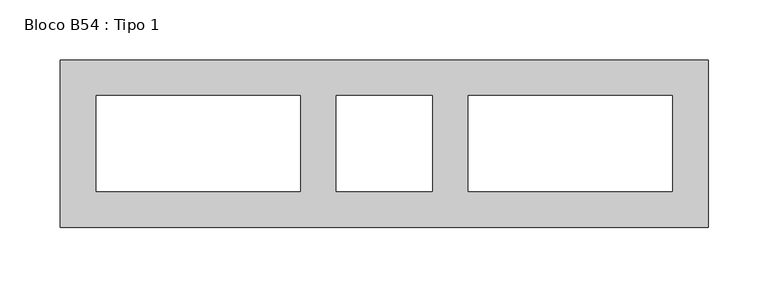
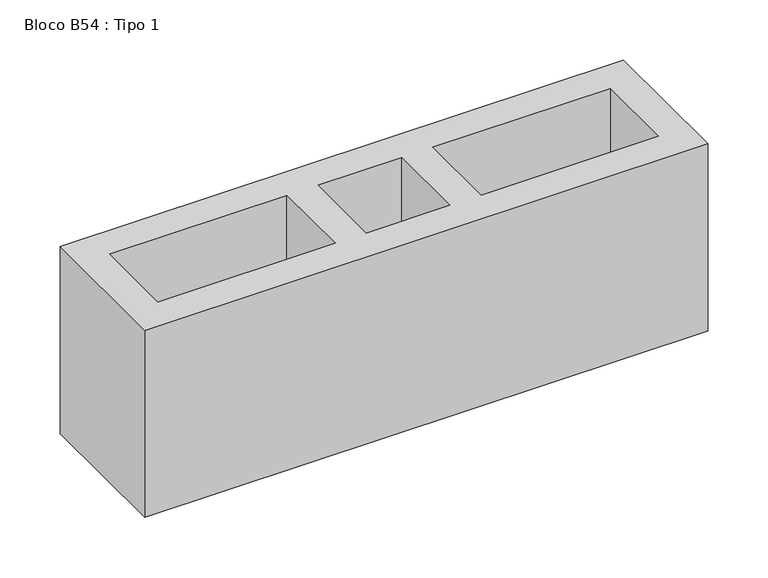
"""IFC4 building model written with IfcOpenShell, lengths in millimetres: proxy geometry, Bloco B54 : Tipo 1."""

from ifc_helpers import new_model, si_unit, origin, origin_with_axes, place, context, project, spatial, polyline, outline, extrude, source, transform, mapped, element, save


def bloco_b54_tipo_1_bdfd0e36(model_context):
    return source(origin(), model_context, "Body", "SweptSolid", [
        extrude(outline(polyline([(540.0, 140.0), (540.0, 0.0), (0.0, 0.0), (0.0, 140.0), (540.0, 140.0)]), holes=[polyline([(340.0, 110.0), (340.0, 30.0), (510.0, 30.0), (510.0, 110.0), (340.0, 110.0)]), polyline([(200.0, 110.0), (30.0, 110.0), (30.0, 30.0), (200.0, 30.0), (200.0, 110.0)]), polyline([(310.0, 110.0), (230.0, 110.0), (230.0, 30.0), (310.0, 30.0), (310.0, 110.0)])]), origin_with_axes(), (0.0, 0.0, 1.0), 190.0),
    ])


if __name__ == "__main__":
    model = new_model("IFC4")
    model_context = context("Model", 3, world=origin())
    ifc_project = project(units=[si_unit("LENGTHUNIT", "METRE", prefix="MILLI")], contexts=[model_context])
    site = spatial("IfcSite", under=ifc_project)
    building = spatial("IfcBuilding", under=site)
    placement = place(None, origin())
    bloco_b54_tipo_1_shape = bloco_b54_tipo_1_bdfd0e36(model_context)
    element("IfcBuildingElementProxy", 1, Name="Bloco B54 : Tipo 1", ObjectType="Bloco B54 : Tipo 1", at=placement, inside=building, context=model_context, shape_type="MappedRepresentation", body=[
        mapped(bloco_b54_tipo_1_shape, transform((0.0, 0.0, 0.0), x_axis=(1.0, 0.0, 0.0), y_axis=(0.0, 1.0, 0.0), z_axis=(0.0, 0.0, 1.0))),
    ])
    save(model, "model.ifc")

# Revit data of these elements
# Type "Bloco B54 : Tipo 1"
#   SINAPI = ""
#   Assembly Code = ""
